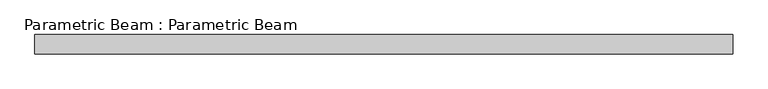
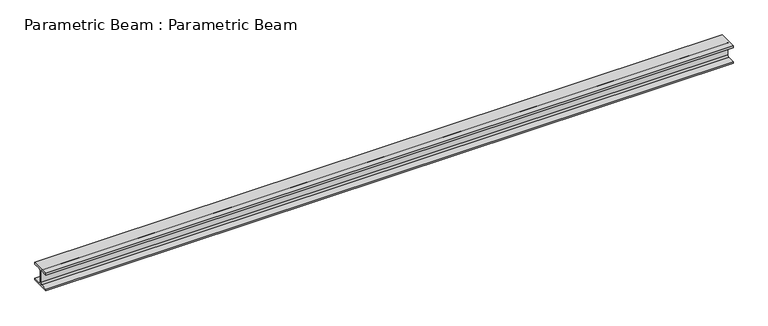
"""IFC4 building model written with IfcOpenShell, lengths in millimetres: beam geometry, Parametric Beam : Parametric Beam."""

from ifc_helpers import new_model, si_unit, point, frame, frame_2d, origin, place, context, project, spatial, polyline, circle_curve, trimmed, segment, composite_curve, outline, extrude, source, transform, mapped, element, save


def parametric_beam_parametric_beam_2c295e66(model_context):
    return source(origin(), model_context, "Body", "SweptSolid", [
        extrude(outline(composite_curve([segment(polyline([(3.75, 72.0), (3.75, -72.0)]), True, "CONTINUOUS"), segment(trimmed(circle_curve(frame_2d((24.75, -72.0)), 21.0), [point((3.75, -72.0))], [point((24.75, -93.0))], True, "CARTESIAN"), True, "CONTINUOUS"), segment(polyline([(24.75, -93.0), (120.0, -93.0), (120.0, -115.0), (-120.0, -115.0), (-120.0, -93.0), (-24.75, -93.0)]), True, "CONTINUOUS"), segment(trimmed(circle_curve(frame_2d((-24.75, -72.0)), 21.0), [point((-24.75, -93.0))], [point((-3.75, -72.0))], True, "CARTESIAN"), True, "CONTINUOUS"), segment(polyline([(-3.75, -72.0), (-3.75, 72.0)]), True, "CONTINUOUS"), segment(trimmed(circle_curve(frame_2d((-24.75, 72.0)), 21.0), [point((-3.75, 72.0))], [point((-24.75, 93.0))], True, "CARTESIAN"), True, "CONTINUOUS"), segment(polyline([(-24.75, 93.0), (-120.0, 93.0), (-120.0, 115.0), (120.0, 115.0), (120.0, 93.0), (24.75, 93.0)]), True, "CONTINUOUS"), segment(trimmed(circle_curve(frame_2d((24.75, 72.0)), 21.0), [point((24.75, 93.0))], [point((3.75, 72.0))], True, "CARTESIAN"), True, "CONTINUOUS")], self_intersect=False)), frame((-4305.243318, 0.0, 0.0), z_axis=(1.0, 0.0, 0.0), x_axis=(0.0, 1.0, 0.0)), (0.0, 0.0, 1.0), 8610.486636),
    ])


if __name__ == "__main__":
    model = new_model("IFC4")
    model_context = context("Model", 3, world=origin())
    ifc_project = project(units=[si_unit("LENGTHUNIT", "METRE", prefix="MILLI")], contexts=[model_context])
    site = spatial("IfcSite", under=ifc_project)
    building = spatial("IfcBuilding", under=site)
    placement = place(None, origin())
    parametric_beam_parametric_beam_shape = parametric_beam_parametric_beam_2c295e66(model_context)
    element("IfcBeam", 1, ObjectType="Parametric Beam : Parametric Beam", at=placement, inside=building, context=model_context, shape_type="MappedRepresentation", body=[
        mapped(parametric_beam_parametric_beam_shape, transform((0.0, 0.0, 0.0), x_axis=(1.0, 0.0, 0.0), y_axis=(0.0, 1.0, 0.0), z_axis=(0.0, 0.0, 1.0))),
    ])
    save(model, "model.ifc")

# Revit data of these elements
# Type "Parametric Beam : Parametric Beam"
#   MHP_PRO_Name [instance default] = "HEA"
#   r [instance default] = 0.021 m
#   h [instance default] = 0.3 m
#   b [instance default] = 0.24 m
#   Tw [instance default] = 0.0075 m
#   Tf [instance default] = 0.012 m
#   Length [instance default] = 3 m
#   Viktor_Change [instance default] = yes
# Element 1 (IfcBeam, "Parametric Beam : Parametric Beam")
#   MHP_PRO_Name = "HEA240"
#   h = 0.23 m
#   Tf = 0.022 m
